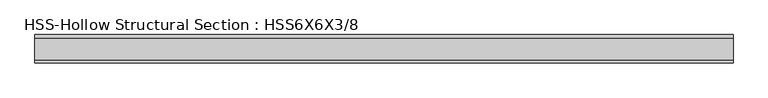
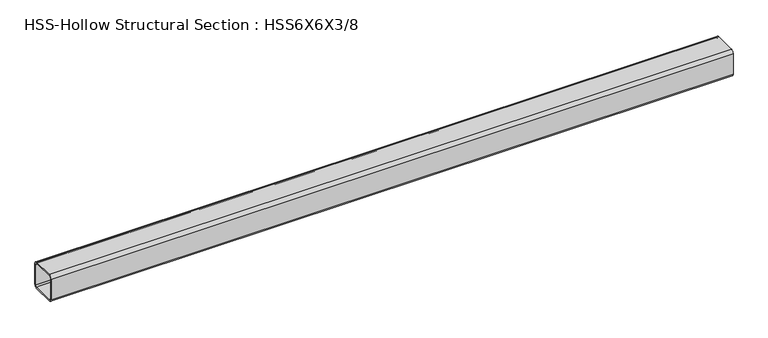
"""IFC4 building model written with IfcOpenShell, lengths in millimetres: member geometry, HSS-Hollow Structural Section : HSS6X6X3/8."""

from ifc_helpers import new_model, si_unit, point, frame, frame_2d, origin, place, context, project, spatial, polyline, circle_curve, trimmed, segment, composite_curve, outline, extrude, source, transform, mapped, element, save


def hss_hollow_structural_section_hss6x6x3_8_6e588ccf(model_context):
    return source(origin(), model_context, "Body", "SweptSolid", [
        extrude(outline(composite_curve([segment(polyline([(76.2, 58.4708), (76.2, -58.4708)]), True, "CONTINUOUS"), segment(trimmed(circle_curve(frame_2d((58.4708, -58.4708)), 17.7292), [point((76.2, -58.4708))], [point((58.4708, -76.2))], False, "CARTESIAN"), True, "CONTINUOUS"), segment(polyline([(58.4708, -76.2), (-58.4708, -76.2)]), True, "CONTINUOUS"), segment(trimmed(circle_curve(frame_2d((-58.4708, -58.4708)), 17.7292), [point((-58.4708, -76.2))], [point((-76.2, -58.4708))], False, "CARTESIAN"), True, "CONTINUOUS"), segment(polyline([(-76.2, -58.4708), (-76.2, 58.4708)]), True, "CONTINUOUS"), segment(trimmed(circle_curve(frame_2d((-58.4708, 58.4708)), 17.7292), [point((-76.2, 58.4708))], [point((-58.4708, 76.2))], False, "CARTESIAN"), True, "CONTINUOUS"), segment(polyline([(-58.4708, 76.2), (58.4708, 76.2)]), True, "CONTINUOUS"), segment(trimmed(circle_curve(frame_2d((58.4708, 58.4708)), 17.7292), [point((58.4708, 76.2))], [point((76.2, 58.4708))], False, "CARTESIAN"), True, "CONTINUOUS")], self_intersect=False), holes=[composite_curve([segment(trimmed(circle_curve(frame_2d((-58.4708, 58.4708)), 8.8646), [point((-58.4708, 67.3354))], [point((-67.3354, 58.4708))], True, "CARTESIAN"), True, "CONTINUOUS"), segment(polyline([(-67.3354, 58.4708), (-67.3354, -58.4708)]), True, "CONTINUOUS"), segment(trimmed(circle_curve(frame_2d((-58.4708, -58.4708)), 8.8646), [point((-67.3354, -58.4708))], [point((-58.4708, -67.3354))], True, "CARTESIAN"), True, "CONTINUOUS"), segment(polyline([(-58.4708, -67.3354), (58.4708, -67.3354)]), True, "CONTINUOUS"), segment(trimmed(circle_curve(frame_2d((58.4708, -58.4708)), 8.8646), [point((58.4708, -67.3354))], [point((67.3354, -58.4708))], True, "CARTESIAN"), True, "CONTINUOUS"), segment(polyline([(67.3354, -58.4708), (67.3354, 58.4708)]), True, "CONTINUOUS"), segment(trimmed(circle_curve(frame_2d((58.4708, 58.4708)), 8.8646), [point((67.3354, 58.4708))], [point((58.4708, 67.3354))], True, "CARTESIAN"), True, "CONTINUOUS"), segment(polyline([(58.4708, 67.3354), (-58.4708, 67.3354)]), True, "CONTINUOUS")], self_intersect=False)]), frame((-1965.3335877, 0.0, 0.0), z_axis=(1.0, 0.0, 0.0), x_axis=(0.0, 1.0, 0.0)), (0.0, 0.0, 1.0), 3725.9173358),
    ])


if __name__ == "__main__":
    model = new_model("IFC4")
    model_context = context("Model", 3, world=origin())
    ifc_project = project(units=[si_unit("LENGTHUNIT", "METRE", prefix="MILLI")], contexts=[model_context])
    site = spatial("IfcSite", under=ifc_project)
    building = spatial("IfcBuilding", under=site)
    placement = place(None, origin())
    hss_hollow_structural_section_hss6x6x3_8_shape = hss_hollow_structural_section_hss6x6x3_8_6e588ccf(model_context)
    element("IfcMember", 1, ObjectType="HSS-Hollow Structural Section : HSS6X6X3/8", at=placement, inside=building, context=model_context, shape_type="MappedRepresentation", body=[
        mapped(hss_hollow_structural_section_hss6x6x3_8_shape, transform((0.0, 0.0, 0.0), x_axis=(1.0, 0.0, 0.0), y_axis=(0.0, 1.0, 0.0), z_axis=(0.0, 0.0, 1.0))),
    ])
    save(model, "model.ifc")

# Revit data of these elements
# Type "HSS-Hollow Structural Section : HSS6X6X3/8"
#   Assembly Code = "B10"
#   Shape = "Square"
#   W = 27.4
#   Ht = 0' - 6"
#   Length [instance default] = 5' - 0"
#   b = 0' - 6"
#   kr = 0' - 0.698"
#   t = 0' - 0.349"
#   A = 0.0526389 SF
#   Structural Material [instance default] = Steel ASTM A500, Grade B, Rectangular and Square
# Element 1 (IfcMember, "HSS-Hollow Structural Section : HSS6X6X3/8")
#   Materials on its faces: "Steel ASTM A500, Grade B, Rectangular and Square"
# Materials
#   "Steel ASTM A500, Grade B, Rectangular and Square": class "Metal", colour RGB 199 199 199, transparency 0, Description = "Carbon steel", Cost = 0
